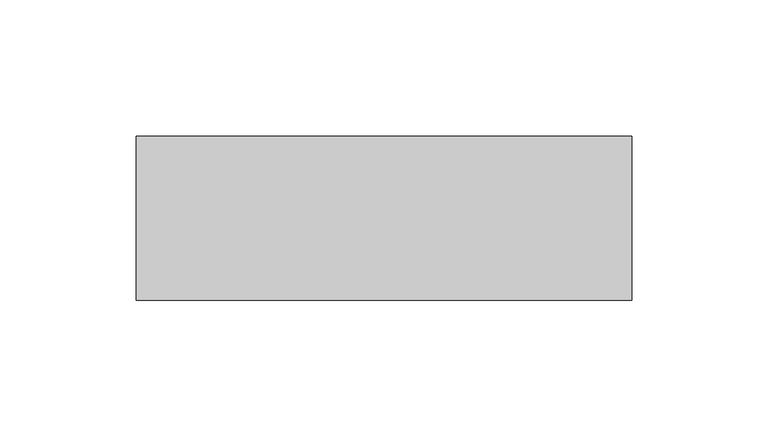
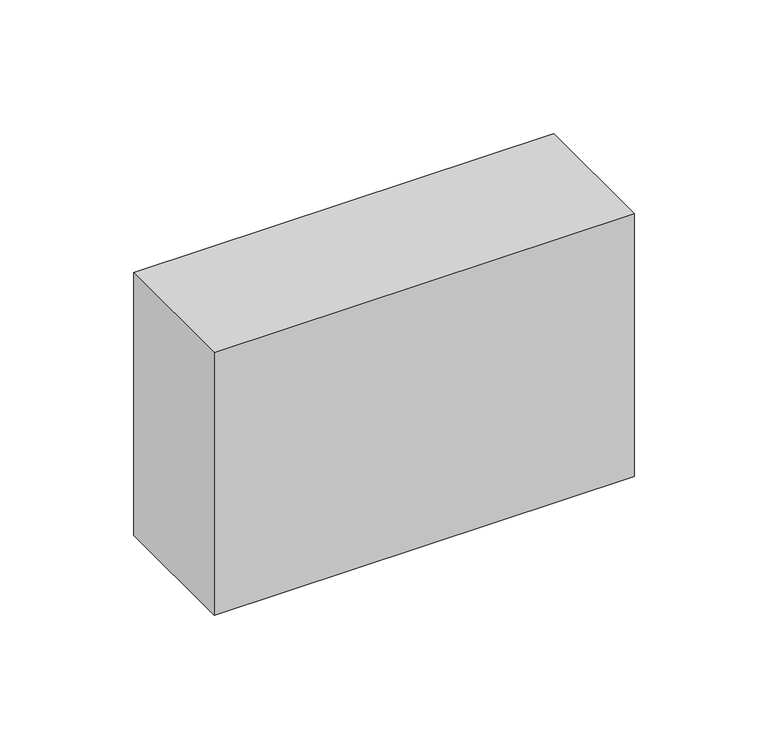
"""IFC4 building model written with IfcOpenShell, lengths in millimetres: beam geometry, Madeira de lei : Berço 6x12cm."""

from ifc_helpers import new_model, si_unit, frame, origin, place, context, project, spatial, polyline, outline, extrude, source, transform, mapped, element, save


def beam_14fb2a3a(model_context):
    return source(origin(), model_context, "Body", "SweptSolid", [
        extrude(outline(polyline([(90.6640427, 30.0), (90.6640427, -30.0), (-90.6640427, -30.0), (-90.6640427, 30.0), (90.6640427, 30.0)])), frame((0.0, 0.0, -60.0), z_axis=(0.0, 0.0, 1.0), x_axis=(1.0, 0.0, 0.0)), (0.0, 0.0, 1.0), 120.0),
    ])


if __name__ == "__main__":
    model = new_model("IFC4")
    model_context = context("Model", 3, world=origin())
    ifc_project = project(units=[si_unit("LENGTHUNIT", "METRE", prefix="MILLI")], contexts=[model_context])
    site = spatial("IfcSite", under=ifc_project)
    building = spatial("IfcBuilding", under=site)
    placement = place(None, origin())
    beam_shape = beam_14fb2a3a(model_context)
    element("IfcBeam", 1, ObjectType="Madeira de lei : Berço 6x12cm", at=placement, inside=building, context=model_context, shape_type="MappedRepresentation", body=[
        mapped(beam_shape, transform((0.0, 0.0, 0.0), x_axis=(1.0, 0.0, 0.0), y_axis=(0.0, 1.0, 0.0), z_axis=(0.0, 0.0, 1.0))),
    ])
    save(model, "model.ifc")

# Revit data of these elements
# Type "Madeira de lei : Berço 6x12cm"
#   A = 0.02 m²
#   Length [instance default] = 1.524 m
#   b = 0.06 m
#   d = 0.12 m
#   Structural Material [instance default] = none
#   Assembly Code = ""
# Element 1 (IfcBeam, "Madeira de lei : Berço 6x12cm")
#   Structural Material = .MADEIRAMENTO
#   Materials on its faces: ".MADEIRAMENTO"
# Materials
#   ".MADEIRAMENTO": class ".CC_MADEIRAS", colour RGB 212 179 113, transparency 0, Cost = 0
